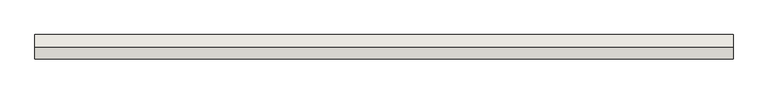
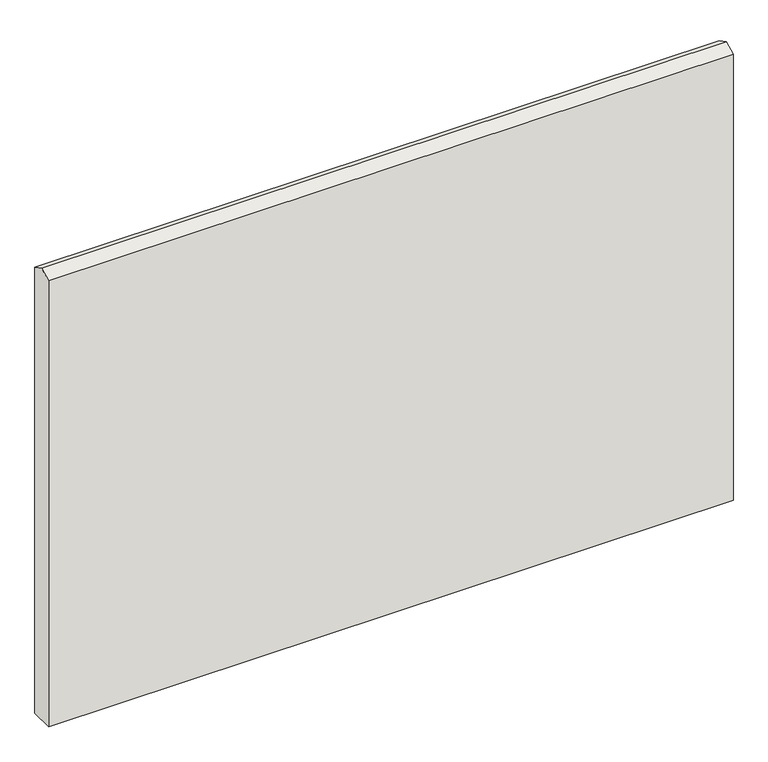
"""IFC4 building model written with IfcOpenShell, lengths in millimetres: wall geometry, Holzwand."""

from ifc_helpers import new_model, si_unit, frame, origin, place, context, project, spatial, polyline, outline, extrude, source, transform, mapped, element, save


def wall_cc1eddbd(model_context):
    return source(origin(), model_context, "Body", "SweptSolid", [
        extrude(outline(polyline([(100.0, 4011.6781465), (200.0, 3960.7256015), (200.0, 0.0), (0.0, 0.0), (0.0, 3960.7256015), (100.0, 4011.6781465)])), frame((0.0, 0.0, 0.0), z_axis=(1.0, 0.0, 0.0), x_axis=(0.0, 1.0, 0.0)), (0.0, 0.0, 1.0), 5750.0),
    ])


if __name__ == "__main__":
    model = new_model("IFC4")
    model_context = context("Model", 3, world=origin())
    ifc_project = project(units=[si_unit("LENGTHUNIT", "METRE", prefix="MILLI")], contexts=[model_context])
    site = spatial("IfcSite", under=ifc_project)
    building = spatial("IfcBuilding", under=site)
    placement = place(None, origin())
    wall_shape = wall_cc1eddbd(model_context)
    element("IfcWall", 1, ObjectType="Holzwand", at=placement, inside=building, context=model_context, shape_type="MappedRepresentation", body=[
        mapped(wall_shape, transform((0.0, 0.0, 0.0), x_axis=(1.0, 0.0, 0.0), y_axis=(0.0, 1.0, 0.0), z_axis=(0.0, 0.0, 1.0))),
    ])
    save(model, "model.ifc")

# Revit data of these elements
# Element 1 (IfcWall, "Holzwand")
#   Materials on its faces: "holzschalung"
# Materials
#   "holzschalung": class "Unassigned", colour RGB 128 128 128, transparency 0
